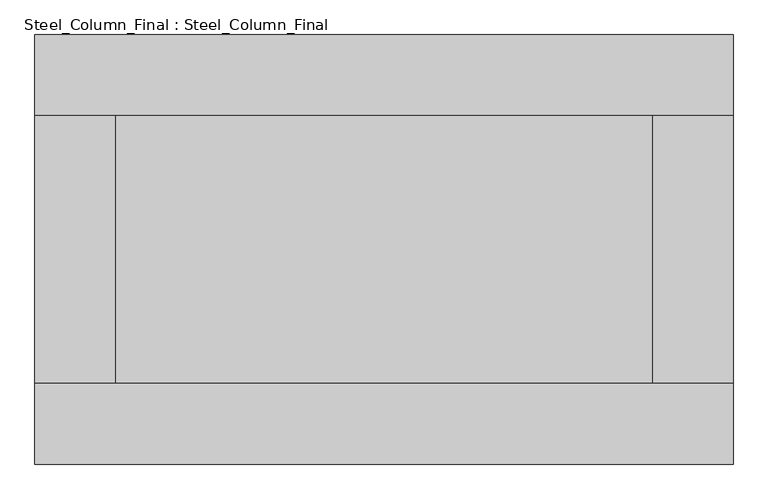
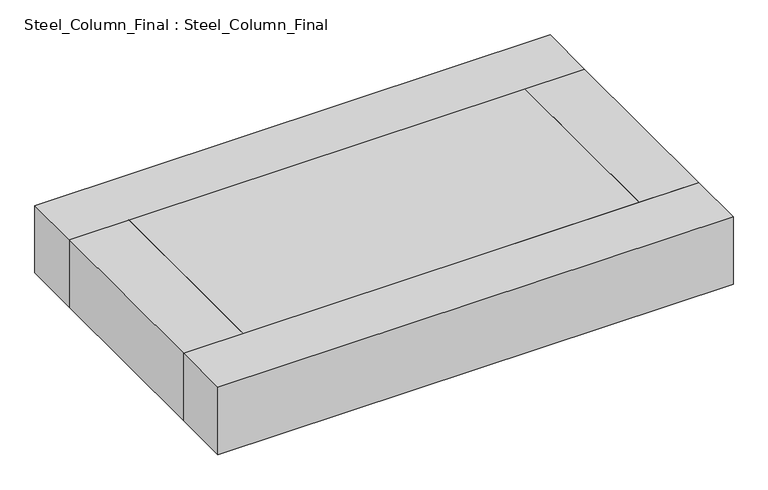
"""IFC4 building model written with IfcOpenShell, lengths in millimetres: proxy geometry, Steel_Column_Final : Steel_Column_Final."""

from ifc_helpers import new_model, si_unit, frame, origin, place, context, project, spatial, polyline, outline, extrude, source, transform, mapped, element, save


def steel_column_final_steel_column_final_07a735ce(model_context):
    return source(origin(), model_context, "Body", "SweptSolid", [
        extrude(outline(polyline([(6500.0, 2500.0), (-6500.0, 2500.0), (-6500.0, 4000.0), (6500.0, 4000.0), (6500.0, 2500.0)])), frame((0.0, 0.0, 22790.0), z_axis=(0.0, 0.0, 1.0), x_axis=(1.0, 0.0, 0.0)), (0.0, 0.0, 1.0), 1800.0),
        extrude(outline(polyline([(-6500.0, -2500.0), (6500.0, -2500.0), (6500.0, -4000.0), (-6500.0, -4000.0), (-6500.0, -2500.0)])), frame((0.0, 0.0, 22790.0), z_axis=(0.0, 0.0, 1.0), x_axis=(1.0, 0.0, 0.0)), (0.0, 0.0, 1.0), 1800.0),
        extrude(outline(polyline([(5000.0, -2500.0), (5000.0, 2500.0), (6500.0, 2500.0), (6500.0, -2500.0), (5000.0, -2500.0)])), frame((0.0, 0.0, 22790.0), z_axis=(0.0, 0.0, 1.0), x_axis=(1.0, 0.0, 0.0)), (0.0, 0.0, 1.0), 1800.0),
        extrude(outline(polyline([(-5000.0, 2500.0), (-5000.0, -2500.0), (-6500.0, -2500.0), (-6500.0, 2500.0), (-5000.0, 2500.0)])), frame((0.0, 0.0, 22790.0), z_axis=(0.0, 0.0, 1.0), x_axis=(1.0, 0.0, 0.0)), (0.0, 0.0, 1.0), 1800.0),
        extrude(outline(polyline([(-5000.0, -2500.0), (-5000.0, 2500.0), (5000.0, 2500.0), (5000.0, -2500.0), (-5000.0, -2500.0)])), frame((0.0, 0.0, 22790.0), z_axis=(0.0, 0.0, 1.0), x_axis=(1.0, 0.0, 0.0)), (0.0, 0.0, 1.0), 1800.0),
    ])


if __name__ == "__main__":
    model = new_model("IFC4")
    model_context = context("Model", 3, world=origin())
    ifc_project = project(units=[si_unit("LENGTHUNIT", "METRE", prefix="MILLI")], contexts=[model_context])
    site = spatial("IfcSite", under=ifc_project)
    building = spatial("IfcBuilding", under=site)
    placement = place(None, origin())
    steel_column_final_steel_column_final_shape = steel_column_final_steel_column_final_07a735ce(model_context)
    element("IfcBuildingElementProxy", 1, Name="Steel_Column_Final : Steel_Column_Final", ObjectType="Steel_Column_Final : Steel_Column_Final", at=placement, inside=building, context=model_context, shape_type="MappedRepresentation", body=[
        mapped(steel_column_final_steel_column_final_shape, transform((0.0, 0.0, 0.0), x_axis=(1.0, 0.0, 0.0), y_axis=(0.0, 1.0, 0.0), z_axis=(0.0, 0.0, 1.0))),
    ])
    save(model, "model.ifc")

# Revit data of these elements
# Type "Steel_Column_Final : Steel_Column_Final"
#   Top Width [instance default] = 5000 mm
#   Top Length = 10000 mm
#   Length = 21000 mm
#   Height [instance default] = 50000 mm
#   Bottom Width [instance default] = 5000 mm
#   Default Elevation = 0
# Element 1 (IfcBuildingElementProxy, "Steel_Column_Final : Steel_Column_Final")
#   Height = 22790 mm
